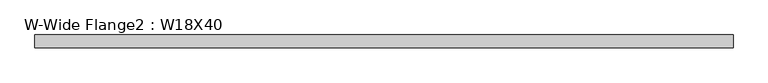
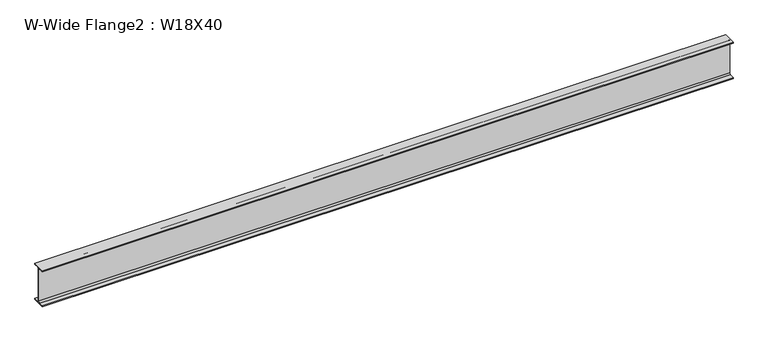
"""IFC4 building model written with IfcOpenShell, lengths in millimetres: beam geometry, W-Wide Flange2 : W18X40."""

import ifcopenshell
import ifcopenshell.guid

model = None  # the IFC model being written
_history = None  # IfcOwnerHistory: only IFC2X3 demands one
_inside = {}  # id of a spatial element -> (the spatial element, [elements in it])
_under = {}  # id of a project, library or spatial element -> (it, [spatial elements below it])
_declared = {}  # id of a project -> (the project, [libraries it declares])
_typed = {}  # id of a type object -> (the type object, [elements of that type])
_made_of = {}  # id of a material, layer set ... -> (it, [elements and type objects made of it])


def new_model(schema):
    """Start an empty IFC model of exactly this schema.

    Asked for "IFC4X3", IfcOpenShell would pick the latest addendum, in which some entities
    have other attributes; the version numbers below select the first issue.
    IFC2X3 requires an IfcOwnerHistory on every rooted entity: one is made here for all.
    """
    global model, _history
    if schema == "IFC4X3":
        model = ifcopenshell.file(schema_version=(4, 3, 0, 0))
    else:
        model = ifcopenshell.file(schema=schema)
    _inside.clear()
    _under.clear()
    _declared.clear()
    _typed.clear()
    _made_of.clear()
    _history = None
    if model.schema == "IFC2X3":
        org = make("IfcOrganization", Name="unknown")
        user = make(
            "IfcPersonAndOrganization",
            ThePerson=make("IfcPerson", FamilyName="unknown"),
            TheOrganization=org,
        )
        app = make(
            "IfcApplication",
            ApplicationDeveloper=org,
            Version="unknown",
            ApplicationFullName="unknown",
            ApplicationIdentifier="unknown",
        )
        _history = make(
            "IfcOwnerHistory",
            OwningUser=user,
            OwningApplication=app,
            ChangeAction="ADDED",
            CreationDate=0,
        )
    return model


def make(cls, **values):
    """One entity of the class cls with the attributes given. An attribute that is None is left unset."""
    return model.create_entity(
        cls, **{name: value for name, value in values.items() if value is not None}
    )


def rooted(cls, **values):
    """An entity with a GlobalId (a new one), such as an element, a storey or a relation."""
    return make(cls, GlobalId=ifcopenshell.guid.new(), OwnerHistory=_history, **values)


def si_unit(unit_type, name, prefix=None):
    """IfcSIUnit, for example si_unit("LENGTHUNIT", "METRE", prefix="MILLI")."""
    return make("IfcSIUnit", UnitType=unit_type, Prefix=prefix, Name=name)


def assignment(units):
    """IfcUnitAssignment: the units of a project."""
    return None if units is None else make("IfcUnitAssignment", Units=units)


def point(xyz):
    """IfcCartesianPoint."""
    return None if xyz is None else make("IfcCartesianPoint", Coordinates=xyz)


def direction(xyz):
    """IfcDirection."""
    return None if xyz is None else make("IfcDirection", DirectionRatios=xyz)


def frame(location, z_axis=None, x_axis=None):
    """IfcAxis2Placement3D, a coordinate frame: its origin and axes. An axis left out is left unset."""
    return make(
        "IfcAxis2Placement3D",
        Location=point(location),
        Axis=direction(z_axis),
        RefDirection=direction(x_axis),
    )


def frame_2d(location, x_axis=None):
    """IfcAxis2Placement2D, a coordinate frame in the plane: its origin and x axis."""
    return make(
        "IfcAxis2Placement2D", Location=point(location), RefDirection=direction(x_axis)
    )


def origin():
    """The frame at (0, 0, 0) with its axes left unset."""
    return frame((0.0, 0.0, 0.0))


def place(relative_to, where):
    """IfcLocalPlacement: puts the frame where relative to a parent placement (None: the world)."""
    return make(
        "IfcLocalPlacement", PlacementRelTo=relative_to, RelativePlacement=where
    )


def context(
    kind, dimensions, precision=None, world=None, true_north=None, identifier=None
):
    """IfcGeometricRepresentationContext, for example the 3D "Model" context."""
    return make(
        "IfcGeometricRepresentationContext",
        ContextIdentifier=identifier,
        ContextType=kind,
        CoordinateSpaceDimension=dimensions,
        Precision=precision,
        WorldCoordinateSystem=world,
        TrueNorth=true_north,
    )


def project(units=None, contexts=None):
    """IfcProject with its units and contexts."""
    return rooted(
        "IfcProject",
        Name="project",
        RepresentationContexts=contexts,
        UnitsInContext=assignment(units),
    )


def spatial(cls, under=None, at=None, **own):
    """A site, building, storey or space (cls), placed at a placement, below another one or the project."""
    s = rooted(cls, ObjectPlacement=at, **own)
    if under is not None:
        _under.setdefault(under.id(), (under, []))[1].append(s)
    return s


def polyline(points):
    """IfcPolyline through the points."""
    return make("IfcPolyline", Points=[point(p) for p in points])


def circle_curve(where, radius):
    """IfcCircle in the frame where."""
    return make("IfcCircle", Position=where, Radius=radius)


def trimmed(basis, trim1, trim2, sense, master):
    """IfcTrimmedCurve: the piece of a basis curve between two trims."""
    return make(
        "IfcTrimmedCurve",
        BasisCurve=basis,
        Trim1=trim1,
        Trim2=trim2,
        SenseAgreement=sense,
        MasterRepresentation=master,
    )


def segment(curve, same_sense, transition):
    """IfcCompositeCurveSegment."""
    return make(
        "IfcCompositeCurveSegment",
        Transition=transition,
        SameSense=same_sense,
        ParentCurve=curve,
    )


def composite_curve(segments, self_intersect=None):
    """IfcCompositeCurve: segments joined end to end."""
    return make("IfcCompositeCurve", Segments=segments, SelfIntersect=self_intersect)


def outline(outer, holes=None, kind="AREA"):
    """IfcArbitraryClosedProfileDef: a profile drawn as a closed curve; with holes, ...WithVoids."""
    if holes is None:
        return make("IfcArbitraryClosedProfileDef", ProfileType=kind, OuterCurve=outer)
    return make(
        "IfcArbitraryProfileDefWithVoids",
        ProfileType=kind,
        OuterCurve=outer,
        InnerCurves=holes,
    )


def extrude(swept, where, along, depth):
    """IfcExtrudedAreaSolid: the profile swept, set in the frame where, extruded along a direction by depth."""
    return make(
        "IfcExtrudedAreaSolid",
        SweptArea=swept,
        Position=where,
        ExtrudedDirection=direction(along),
        Depth=depth,
    )


def shape(context_of_items, identifier, shape_type, items):
    """IfcShapeRepresentation: the items that make up one representation, for example the "Body"."""
    return make(
        "IfcShapeRepresentation",
        ContextOfItems=context_of_items,
        RepresentationIdentifier=identifier,
        RepresentationType=shape_type,
        Items=items,
    )


def source(mapping_origin, context_of_items, identifier, shape_type, items):
    """IfcRepresentationMap: a shape defined once, which mapped items show again and again."""
    return make(
        "IfcRepresentationMap",
        MappingOrigin=mapping_origin,
        MappedRepresentation=shape(context_of_items, identifier, shape_type, items),
    )


def transform(
    local_origin,
    x_axis=None,
    y_axis=None,
    z_axis=None,
    scale=None,
    scale2=None,
    scale3=None,
    uniform=True,
):
    """IfcCartesianTransformationOperator3D, or its non-uniform kind. x_axis, y_axis, z_axis: its Axis1, 2, 3."""
    if uniform:
        return make(
            "IfcCartesianTransformationOperator3D",
            Axis1=direction(x_axis),
            Axis2=direction(y_axis),
            LocalOrigin=point(local_origin),
            Scale=scale,
            Axis3=direction(z_axis),
        )
    return make(
        "IfcCartesianTransformationOperator3DnonUniform",
        Axis1=direction(x_axis),
        Axis2=direction(y_axis),
        LocalOrigin=point(local_origin),
        Scale=scale,
        Axis3=direction(z_axis),
        Scale2=scale2,
        Scale3=scale3,
    )


def mapped(mapping_source, mapping_target):
    """IfcMappedItem: shows the shape of a source again, moved by a transform."""
    return make(
        "IfcMappedItem", MappingSource=mapping_source, MappingTarget=mapping_target
    )


def made_of(thing, what):
    """Note that an element or type object is made of a material, layer set ...; save() writes the relation."""
    if what is not None:
        _made_of.setdefault(what.id(), (what, []))[1].append(thing)
    return thing


def element(
    cls,
    number,
    at=None,
    inside=None,
    cuts=None,
    type_object=None,
    material=None,
    context=None,
    identifier="Body",
    shape_type=None,
    held_by="IfcProductDefinitionShape",
    body=None,
    shapes=None,
    **own,
):
    """One element of the class cls, such as IfcWall. Its Tag is "e" and its number.

    at: its placement. inside: the storey or other place that contains it. cuts: it is an
    opening in that element (IfcRelVoidsElement). A single representation is given by context,
    identifier, shape_type and body (its items); several are given by shapes. held_by: the class
    of the entity that holds the representations. save() writes the other relations.
    """
    e = rooted(cls, Tag="e%d" % number, ObjectPlacement=at, **own)
    if body is not None:
        shapes = [shape(context, identifier, shape_type, body)]
    if shapes is not None:
        e.Representation = make(held_by, Representations=shapes)
    if inside is not None:
        _inside.setdefault(inside.id(), (inside, []))[1].append(e)
    if cuts is not None:
        rooted(
            "IfcRelVoidsElement", RelatingBuildingElement=cuts, RelatedOpeningElement=e
        )
    if type_object is not None:
        _typed.setdefault(type_object.id(), (type_object, []))[1].append(e)
    return made_of(e, material)


def aggregate(whole, parts):
    """IfcRelAggregates: a whole, such as a stair, and the parts it consists of."""
    return rooted("IfcRelAggregates", RelatingObject=whole, RelatedObjects=parts)


def save(model, path):
    """Write the relations noted so far, then the file.

    IfcRelAggregates (storeys below a building ...), IfcRelContainedInSpatialStructure (elements
    in a storey), IfcRelDefinesByType, IfcRelAssociatesMaterial and IfcRelDeclares: one each for
    every whole, place, type object, material and project.
    """
    for whole, parts in _under.values():
        aggregate(whole, parts)
    for where, things in _inside.values():
        rooted(
            "IfcRelContainedInSpatialStructure",
            RelatedElements=things,
            RelatingStructure=where,
        )
    for kind, things in _typed.values():
        rooted("IfcRelDefinesByType", RelatedObjects=things, RelatingType=kind)
    for what, things in _made_of.values():
        rooted("IfcRelAssociatesMaterial", RelatedObjects=things, RelatingMaterial=what)
    for by, libraries in _declared.values():
        rooted("IfcRelDeclares", RelatingContext=by, RelatedDefinitions=libraries)
    model.write(path)


def w_wide_flange2_w18x40_41391f11(model_context):
    return source(origin(), model_context, "Body", "SweptSolid", [
        extrude(outline(composite_curve([segment(polyline([(76.454, -213.995), (76.454, -227.33), (-76.454, -227.33), (-76.454, -213.995), (-20.828, -213.995)]), True, "CONTINUOUS"), segment(trimmed(circle_curve(frame_2d((-20.828, -197.1675)), 16.8275), [point((-20.828, -213.995))], [point((-4.0005, -197.1675))], True, "CARTESIAN"), True, "CONTINUOUS"), segment(polyline([(-4.0005, -197.1675), (-4.0005, 197.1675)]), True, "CONTINUOUS"), segment(trimmed(circle_curve(frame_2d((-20.828, 197.1675)), 16.8275), [point((-4.0005, 197.1675))], [point((-20.828, 213.995))], True, "CARTESIAN"), True, "CONTINUOUS"), segment(polyline([(-20.828, 213.995), (-76.454, 213.995), (-76.454, 227.33), (76.454, 227.33), (76.454, 213.995), (20.828, 213.995)]), True, "CONTINUOUS"), segment(trimmed(circle_curve(frame_2d((20.828, 197.1675)), 16.8275), [point((20.828, 213.995))], [point((4.0005, 197.1675))], True, "CARTESIAN"), True, "CONTINUOUS"), segment(polyline([(4.0005, 197.1675), (4.0005, -197.1675)]), True, "CONTINUOUS"), segment(trimmed(circle_curve(frame_2d((20.828, -197.1675)), 16.8275), [point((4.0005, -197.1675))], [point((20.828, -213.995))], True, "CARTESIAN"), True, "CONTINUOUS"), segment(polyline([(20.828, -213.995), (76.454, -213.995)]), True, "CONTINUOUS")], self_intersect=False)), frame((-4095.353125, 0.0, 0.0), z_axis=(1.0, 0.0, 0.0), x_axis=(0.0, 1.0, 0.0)), (0.0, 0.0, 1.0), 8190.70625),
    ])


if __name__ == "__main__":
    model = new_model("IFC4")
    model_context = context("Model", 3, world=origin())
    ifc_project = project(units=[si_unit("LENGTHUNIT", "METRE", prefix="MILLI")], contexts=[model_context])
    site = spatial("IfcSite", under=ifc_project)
    building = spatial("IfcBuilding", under=site)
    placement = place(None, origin())
    w_wide_flange2_w18x40_shape = w_wide_flange2_w18x40_41391f11(model_context)
    element("IfcBeam", 1, ObjectType="W-Wide Flange2 : W18X40", at=placement, inside=building, context=model_context, shape_type="MappedRepresentation", body=[
        mapped(w_wide_flange2_w18x40_shape, transform((0.0, 0.0, 0.0), x_axis=(1.0, 0.0, 0.0), y_axis=(0.0, 1.0, 0.0), z_axis=(0.0, 0.0, 1.0))),
    ])
    save(model, "model.ifc")

# Revit data of these elements
# Type "W-Wide Flange2 : W18X40"
#   Assembly Code = "B10"
#   W = 40
#   Length [instance default] = 5' - 0"
#   bf = 0' - 6.02"
#   d = 1' - 5.9"
#   k = 0' - 1 3/16"
#   k2 = 0' - 0.6625"
#   tf = 0' - 0.525"
#   tw = 0' - 0.315"
#   A = 0.0819444 SF
#   Structural Material [instance default] = Steel ASTM A992
# Element 1 (IfcBeam, "W-Wide Flange2 : W18X40")
#   Materials on its faces: "Steel ASTM A992"
# Materials
#   "Steel ASTM A992": class "Metal", colour RGB 199 199 199, transparency 0, Description = "Structural steel 50ksi", Cost = 0
